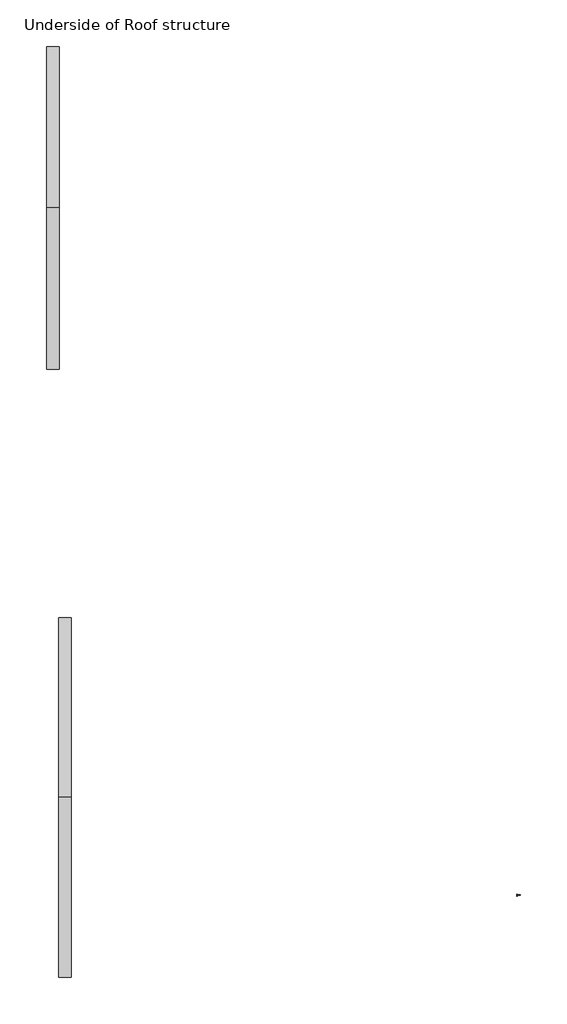
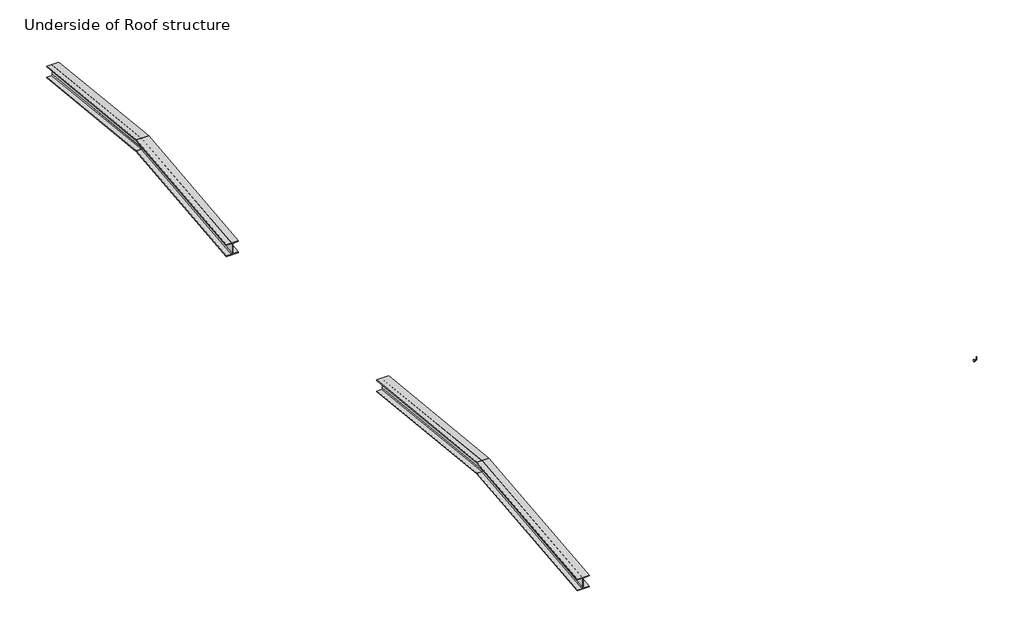
# One storey: 4 beams, 1 proxy.
"""IFC4 building model written with IfcOpenShell, lengths in millimetres."""

import ifcopenshell
import ifcopenshell.guid

model = None  # the IFC model being written
_history = None  # IfcOwnerHistory: only IFC2X3 demands one
_inside = {}  # id of a spatial element -> (the spatial element, [elements in it])
_under = {}  # id of a project, library or spatial element -> (it, [spatial elements below it])
_declared = {}  # id of a project -> (the project, [libraries it declares])
_typed = {}  # id of a type object -> (the type object, [elements of that type])
_made_of = {}  # id of a material, layer set ... -> (it, [elements and type objects made of it])


def new_model(schema):
    """Start an empty IFC model of exactly this schema.

    Asked for "IFC4X3", IfcOpenShell would pick the latest addendum, in which some entities
    have other attributes; the version numbers below select the first issue.
    IFC2X3 requires an IfcOwnerHistory on every rooted entity: one is made here for all.
    """
    global model, _history
    if schema == "IFC4X3":
        model = ifcopenshell.file(schema_version=(4, 3, 0, 0))
    else:
        model = ifcopenshell.file(schema=schema)
    _inside.clear()
    _under.clear()
    _declared.clear()
    _typed.clear()
    _made_of.clear()
    _history = None
    if model.schema == "IFC2X3":
        org = make("IfcOrganization", Name="unknown")
        user = make(
            "IfcPersonAndOrganization",
            ThePerson=make("IfcPerson", FamilyName="unknown"),
            TheOrganization=org,
        )
        app = make(
            "IfcApplication",
            ApplicationDeveloper=org,
            Version="unknown",
            ApplicationFullName="unknown",
            ApplicationIdentifier="unknown",
        )
        _history = make(
            "IfcOwnerHistory",
            OwningUser=user,
            OwningApplication=app,
            ChangeAction="ADDED",
            CreationDate=0,
        )
    return model


def make(cls, **values):
    """One entity of the class cls with the attributes given. An attribute that is None is left unset."""
    return model.create_entity(
        cls, **{name: value for name, value in values.items() if value is not None}
    )


def rooted(cls, **values):
    """An entity with a GlobalId (a new one), such as an element, a storey or a relation."""
    return make(cls, GlobalId=ifcopenshell.guid.new(), OwnerHistory=_history, **values)


def si_unit(unit_type, name, prefix=None):
    """IfcSIUnit, for example si_unit("LENGTHUNIT", "METRE", prefix="MILLI")."""
    return make("IfcSIUnit", UnitType=unit_type, Prefix=prefix, Name=name)


def assignment(units):
    """IfcUnitAssignment: the units of a project."""
    return None if units is None else make("IfcUnitAssignment", Units=units)


def point(xyz):
    """IfcCartesianPoint."""
    return None if xyz is None else make("IfcCartesianPoint", Coordinates=xyz)


def direction(xyz):
    """IfcDirection."""
    return None if xyz is None else make("IfcDirection", DirectionRatios=xyz)


def frame(location, z_axis=None, x_axis=None):
    """IfcAxis2Placement3D, a coordinate frame: its origin and axes. An axis left out is left unset."""
    return make(
        "IfcAxis2Placement3D",
        Location=point(location),
        Axis=direction(z_axis),
        RefDirection=direction(x_axis),
    )


def frame_2d(location, x_axis=None):
    """IfcAxis2Placement2D, a coordinate frame in the plane: its origin and x axis."""
    return make(
        "IfcAxis2Placement2D", Location=point(location), RefDirection=direction(x_axis)
    )


def origin():
    """The frame at (0, 0, 0) with its axes left unset."""
    return frame((0.0, 0.0, 0.0))


def origin_with_axes():
    """The frame at (0, 0, 0) with the z axis (0, 0, 1) and the x axis (1, 0, 0) written out."""
    return frame((0.0, 0.0, 0.0), z_axis=(0.0, 0.0, 1.0), x_axis=(1.0, 0.0, 0.0))


def place(relative_to, where):
    """IfcLocalPlacement: puts the frame where relative to a parent placement (None: the world)."""
    return make(
        "IfcLocalPlacement", PlacementRelTo=relative_to, RelativePlacement=where
    )


def context(
    kind, dimensions, precision=None, world=None, true_north=None, identifier=None
):
    """IfcGeometricRepresentationContext, for example the 3D "Model" context."""
    return make(
        "IfcGeometricRepresentationContext",
        ContextIdentifier=identifier,
        ContextType=kind,
        CoordinateSpaceDimension=dimensions,
        Precision=precision,
        WorldCoordinateSystem=world,
        TrueNorth=true_north,
    )


def project(units=None, contexts=None):
    """IfcProject with its units and contexts."""
    return rooted(
        "IfcProject",
        Name="project",
        RepresentationContexts=contexts,
        UnitsInContext=assignment(units),
    )


def spatial(cls, under=None, at=None, **own):
    """A site, building, storey or space (cls), placed at a placement, below another one or the project."""
    s = rooted(cls, ObjectPlacement=at, **own)
    if under is not None:
        _under.setdefault(under.id(), (under, []))[1].append(s)
    return s


def polyline(points):
    """IfcPolyline through the points."""
    return make("IfcPolyline", Points=[point(p) for p in points])


def circle_curve(where, radius):
    """IfcCircle in the frame where."""
    return make("IfcCircle", Position=where, Radius=radius)


def ellipse_curve(where, semi_axis1, semi_axis2):
    """IfcEllipse in the frame where."""
    return make(
        "IfcEllipse", Position=where, SemiAxis1=semi_axis1, SemiAxis2=semi_axis2
    )


def trimmed(basis, trim1, trim2, sense, master):
    """IfcTrimmedCurve: the piece of a basis curve between two trims."""
    return make(
        "IfcTrimmedCurve",
        BasisCurve=basis,
        Trim1=trim1,
        Trim2=trim2,
        SenseAgreement=sense,
        MasterRepresentation=master,
    )


def segment(curve, same_sense, transition):
    """IfcCompositeCurveSegment."""
    return make(
        "IfcCompositeCurveSegment",
        Transition=transition,
        SameSense=same_sense,
        ParentCurve=curve,
    )


def composite_curve(segments, self_intersect=None):
    """IfcCompositeCurve: segments joined end to end."""
    return make("IfcCompositeCurve", Segments=segments, SelfIntersect=self_intersect)


def outline(outer, holes=None, kind="AREA"):
    """IfcArbitraryClosedProfileDef: a profile drawn as a closed curve; with holes, ...WithVoids."""
    if holes is None:
        return make("IfcArbitraryClosedProfileDef", ProfileType=kind, OuterCurve=outer)
    return make(
        "IfcArbitraryProfileDefWithVoids",
        ProfileType=kind,
        OuterCurve=outer,
        InnerCurves=holes,
    )


def extrude(swept, where, along, depth):
    """IfcExtrudedAreaSolid: the profile swept, set in the frame where, extruded along a direction by depth."""
    return make(
        "IfcExtrudedAreaSolid",
        SweptArea=swept,
        Position=where,
        ExtrudedDirection=direction(along),
        Depth=depth,
    )


def shape(context_of_items, identifier, shape_type, items):
    """IfcShapeRepresentation: the items that make up one representation, for example the "Body"."""
    return make(
        "IfcShapeRepresentation",
        ContextOfItems=context_of_items,
        RepresentationIdentifier=identifier,
        RepresentationType=shape_type,
        Items=items,
    )


def source(mapping_origin, context_of_items, identifier, shape_type, items):
    """IfcRepresentationMap: a shape defined once, which mapped items show again and again."""
    return make(
        "IfcRepresentationMap",
        MappingOrigin=mapping_origin,
        MappedRepresentation=shape(context_of_items, identifier, shape_type, items),
    )


def transform(
    local_origin,
    x_axis=None,
    y_axis=None,
    z_axis=None,
    scale=None,
    scale2=None,
    scale3=None,
    uniform=True,
):
    """IfcCartesianTransformationOperator3D, or its non-uniform kind. x_axis, y_axis, z_axis: its Axis1, 2, 3."""
    if uniform:
        return make(
            "IfcCartesianTransformationOperator3D",
            Axis1=direction(x_axis),
            Axis2=direction(y_axis),
            LocalOrigin=point(local_origin),
            Scale=scale,
            Axis3=direction(z_axis),
        )
    return make(
        "IfcCartesianTransformationOperator3DnonUniform",
        Axis1=direction(x_axis),
        Axis2=direction(y_axis),
        LocalOrigin=point(local_origin),
        Scale=scale,
        Axis3=direction(z_axis),
        Scale2=scale2,
        Scale3=scale3,
    )


def mapped(mapping_source, mapping_target):
    """IfcMappedItem: shows the shape of a source again, moved by a transform."""
    return make(
        "IfcMappedItem", MappingSource=mapping_source, MappingTarget=mapping_target
    )


def made_of(thing, what):
    """Note that an element or type object is made of a material, layer set ...; save() writes the relation."""
    if what is not None:
        _made_of.setdefault(what.id(), (what, []))[1].append(thing)
    return thing


def element(
    cls,
    number,
    at=None,
    inside=None,
    cuts=None,
    type_object=None,
    material=None,
    context=None,
    identifier="Body",
    shape_type=None,
    held_by="IfcProductDefinitionShape",
    body=None,
    shapes=None,
    **own,
):
    """One element of the class cls, such as IfcWall. Its Tag is "e" and its number.

    at: its placement. inside: the storey or other place that contains it. cuts: it is an
    opening in that element (IfcRelVoidsElement). A single representation is given by context,
    identifier, shape_type and body (its items); several are given by shapes. held_by: the class
    of the entity that holds the representations. save() writes the other relations.
    """
    e = rooted(cls, Tag="e%d" % number, ObjectPlacement=at, **own)
    if body is not None:
        shapes = [shape(context, identifier, shape_type, body)]
    if shapes is not None:
        e.Representation = make(held_by, Representations=shapes)
    if inside is not None:
        _inside.setdefault(inside.id(), (inside, []))[1].append(e)
    if cuts is not None:
        rooted(
            "IfcRelVoidsElement", RelatingBuildingElement=cuts, RelatedOpeningElement=e
        )
    if type_object is not None:
        _typed.setdefault(type_object.id(), (type_object, []))[1].append(e)
    return made_of(e, material)


def aggregate(whole, parts):
    """IfcRelAggregates: a whole, such as a stair, and the parts it consists of."""
    return rooted("IfcRelAggregates", RelatingObject=whole, RelatedObjects=parts)


def save(model, path):
    """Write the relations noted so far, then the file.

    IfcRelAggregates (storeys below a building ...), IfcRelContainedInSpatialStructure (elements
    in a storey), IfcRelDefinesByType, IfcRelAssociatesMaterial and IfcRelDeclares: one each for
    every whole, place, type object, material and project.
    """
    for whole, parts in _under.values():
        aggregate(whole, parts)
    for where, things in _inside.values():
        rooted(
            "IfcRelContainedInSpatialStructure",
            RelatedElements=things,
            RelatingStructure=where,
        )
    for kind, things in _typed.values():
        rooted("IfcRelDefinesByType", RelatedObjects=things, RelatingType=kind)
    for what, things in _made_of.values():
        rooted("IfcRelAssociatesMaterial", RelatedObjects=things, RelatingMaterial=what)
    for by, libraries in _declared.values():
        rooted("IfcRelDeclares", RelatingContext=by, RelatedDefinitions=libraries)
    model.write(path)


def plane_surface(at):
    """IfcPlane: the flat surface through the origin of the frame at, square to its z axis."""
    return make("IfcPlane", Position=at)


def cylinder_surface(at, radius):
    """IfcCylindricalSurface: all points at the distance radius from the z axis of the frame at."""
    return make("IfcCylindricalSurface", Position=at, Radius=radius)


def revolved_surface(curve, axis_point, axis_direction):
    """IfcSurfaceOfRevolution: the curve turned about the line through axis_point along axis_direction."""
    return make(
        "IfcSurfaceOfRevolution",
        SweptCurve=make("IfcArbitraryOpenProfileDef", ProfileType="CURVE", Curve=curve),
        AxisPosition=make("IfcAxis1Placement", Location=point(axis_point), Axis=direction(axis_direction)),
    )


def advanced_brep(points, edges, surfaces, faces):
    """IfcAdvancedBrep: a solid bounded by faces that lie on surfaces and meet in shared edges.

    An edge is (start, end): straight between two places in points (the first is 0);
    or (start, end, curve); or (start, end, curve, False) where it runs against its curve.
    A face is (place in surfaces, loops), or (place, loops, False) where it looks against
    its surface's normal. A loop lists edges by number (the first is 1), with a minus sign
    where the edge is run from its end to its start. The first loop is the outer one.
    """
    corners = [point(p) for p in points]
    vertices = [make("IfcVertexPoint", VertexGeometry=c) for c in corners]
    made = []
    for start, end, *more in edges:
        made.append(
            make(
                "IfcEdgeCurve",
                EdgeStart=vertices[start],
                EdgeEnd=vertices[end],
                EdgeGeometry=more[0] if more else make("IfcPolyline", Points=[corners[start], corners[end]]),
                SameSense=more[1] if len(more) > 1 else True,
            )
        )
    hull = []
    for where, loops, *sense in faces:
        bounds = []
        for j, loop in enumerate(loops):
            ring = [make("IfcOrientedEdge", EdgeElement=made[abs(k) - 1], Orientation=k > 0) for k in loop]
            bounds.append(
                make(
                    "IfcFaceOuterBound" if j == 0 else "IfcFaceBound",
                    Bound=make("IfcEdgeLoop", EdgeList=ring),
                    Orientation=True,
                )
            )
        hull.append(make("IfcAdvancedFace", Bounds=bounds, FaceSurface=surfaces[where], SameSense=sense[0] if sense else True))
    return make("IfcAdvancedBrep", Outer=make("IfcClosedShell", CfsFaces=hull))


def support_metal_circular1_support_metal_circular_6fb01533(model_context):
    return source(origin(), model_context, "Body", "SolidModel", [
        advanced_brep(
        [(0.0, 63.5, -69.85), (0.0, 63.5, -82.55), (0.0, 12.7, -69.85), (0.0, 12.7, -82.55), (0.0, -6.35, -63.5), (0.0, 6.35, -63.5), (0.0, 6.35, 0.0), (0.0, -6.35, 0.0)],
        [
            (0, 1, circle_curve(frame((0.0, 63.5, -76.2), z_axis=(0.0, 1.0, 0.0), x_axis=(0.0, 0.0, -1.0)), 6.35)),
            (1, 0, circle_curve(frame((0.0, 63.5, -76.2), z_axis=(0.0, 1.0, 0.0), x_axis=(0.0, 0.0, -1.0)), 6.35)),
            (0, 2),
            (2, 3, circle_curve(frame((0.0, 12.7, -76.2), z_axis=(0.0, 1.0, 0.0), x_axis=(0.0, 0.0, -1.0)), 6.35)),
            (3, 1),
            (3, 2, circle_curve(frame((0.0, 12.7, -76.2), z_axis=(0.0, 1.0, 0.0), x_axis=(0.0, 0.0, -1.0)), 6.35)),
            (4, 3, circle_curve(frame((0.0, 12.7, -63.5), z_axis=(1.0, 0.0, 0.0), x_axis=(0.0, 0.0, -1.0)), 19.05)),
            (2, 5, circle_curve(frame((0.0, 12.7, -63.5), z_axis=(-1.0, 0.0, 0.0), x_axis=(0.0, 0.0, -1.0)), 6.35)),
            (5, 4, circle_curve(frame((0.0, 0.0, -63.5), z_axis=(0.0, 0.0, -1.0), x_axis=(0.0, -1.0, 0.0)), 6.35)),
            (4, 5, circle_curve(frame((0.0, 0.0, -63.5), z_axis=(0.0, 0.0, -1.0), x_axis=(0.0, -1.0, 0.0)), 6.35)),
            (6, 7, circle_curve(frame((0.0, 0.0, 0.0), z_axis=(0.0, 0.0, 1.0), x_axis=(0.0, -1.0, 0.0)), 6.35)),
            (7, 6, circle_curve(frame((0.0, 0.0, 0.0), z_axis=(0.0, 0.0, 1.0), x_axis=(0.0, -1.0, 0.0)), 6.35)),
            (5, 6),
            (7, 4),
        ],
        [
            plane_surface(frame((0.0, 63.5, -76.2), z_axis=(0.0, 1.0, 0.0), x_axis=(1.0, 0.0, 0.0))),
            cylinder_surface(frame((0.0, 63.5, -76.2), z_axis=(0.0, 1.0, 0.0), x_axis=(0.0, 0.0, -1.0)), 6.35),
            revolved_surface(trimmed(ellipse_curve(frame((0.0, 12.7, -76.2), z_axis=(0.0, 1.0, 0.0), x_axis=(0.0, 0.0, -1.0)), 6.35, 6.35), [point((0.0, 12.7, -69.85))], [point((0.0, 12.7, -82.55))], True, "CARTESIAN"), (0.0, 12.7, -63.5), (-1.0, 0.0, 0.0)),
            revolved_surface(trimmed(ellipse_curve(frame((0.0, 12.7, -76.2), z_axis=(0.0, 1.0, 0.0), x_axis=(0.0, 0.0, -1.0)), 6.35, 6.35), [point((0.0, 12.7, -82.55))], [point((0.0, 12.7, -69.85))], True, "CARTESIAN"), (0.0, 12.7, -63.5), (-1.0, 0.0, 0.0)),
            plane_surface(origin_with_axes()),
            cylinder_surface(frame((0.0, 0.0, -63.5), z_axis=(0.0, 0.0, -1.0), x_axis=(0.0, -1.0, 0.0)), 6.35),
        ],
        [
            (0, [[1, 2]]),
            (1, [[-1, 3, 4, 5]]),
            (1, [[-2, -5, 6, -3]]),
            (2, [[7, -4, 8, 9]]),
            (3, [[-8, -6, -7, 10]]),
            (4, [[11, 12]]),
            (5, [[-9, 13, -12, 14]]),
            (5, [[-10, -14, -11, -13]]),
        ],
    ),
        extrude(outline(composite_curve([segment(trimmed(circle_curve(frame_2d((-76.2, 0.0)), 25.4), [point((-76.2, -25.4))], [point((-76.2, 25.4))], False, "CARTESIAN"), True, "CONTINUOUS"), segment(trimmed(circle_curve(frame_2d((-76.2, 0.0)), 25.4), [point((-76.2, 25.4))], [point((-76.2, -25.4))], False, "CARTESIAN"), True, "CONTINUOUS")], self_intersect=False)), frame((0.0, 63.5, 0.0), z_axis=(0.0, 1.0, 0.0), x_axis=(0.0, 0.0, 1.0)), (0.0, 0.0, 1.0), 12.7),
    ])


model = new_model("IFC4")

# Units and contexts
model_context = context("Model", 3, world=origin())
ifc_project = project(units=[si_unit("LENGTHUNIT", "METRE", prefix="MILLI")], contexts=[model_context])

# Site, building, storey
site = spatial("IfcSite", under=ifc_project)
building = spatial("IfcBuilding", under=site)
storey = spatial("IfcBuildingStorey", under=building, Name="Underside of Roof structure", Elevation=34036.0)

# Beams
placement = place(None, origin())
element("IfcBeam", 1, ObjectType="W-Wide Flange : W12X79", at=placement, inside=storey, context=model_context, shape_type="AdvancedBrep", body=[
    advanced_brep(
    [(-21755.4154607, 20844.8695005, 33191.9562864), (-21630.3204607, 20844.8695005, 33191.9562864), (-21607.7144607, 20844.8695005, 33214.6883829), (-21607.7144607, 20844.8695005, 33448.3947677), (-21630.3204607, 20844.8695005, 33471.1268642), (-21755.4154607, 20844.8695005, 33471.1268642), (-21755.4154607, 20844.8695005, 33489.9), (-21448.0754607, 20844.8695005, 33489.9), (-21448.0754607, 20844.8695005, 33471.1268642), (-21573.1704607, 20844.8695005, 33471.1268642), (-21595.7764607, 20844.8695005, 33448.3947677), (-21595.7764607, 20844.8695005, 33214.6883829), (-21573.1704607, 20844.8695005, 33191.9562864), (-21448.0754607, 20844.8695005, 33191.9562864), (-21448.0754607, 20844.8695005, 33173.1831506), (-21755.4154607, 20844.8695005, 33173.1831506), (-21755.4154607, 16882.4695005, 33611.0562864), (-21630.3204607, 16882.4695005, 33611.0562864), (-21755.4154607, 16882.4695005, 33592.2831506), (-21448.0754607, 16882.4695005, 33592.2831506), (-21448.0754607, 16882.4695005, 33611.0562864), (-21573.1704607, 16882.4695005, 33611.0562864), (-21595.7764607, 16882.4695005, 33633.7883829), (-21595.7764607, 16882.4695005, 33867.4947677), (-21573.1704607, 16882.4695005, 33890.2268642), (-21448.0754607, 16882.4695005, 33890.2268642), (-21448.0754607, 16882.4695005, 33909.0), (-21755.4154607, 16882.4695005, 33909.0), (-21755.4154607, 16882.4695005, 33890.2268642), (-21630.3204607, 16882.4695005, 33890.2268642), (-21607.7144607, 16882.4695005, 33867.4947677), (-21607.7144607, 16882.4695005, 33633.7883829)],
    [
        (0, 1),
        (1, 2, ellipse_curve(frame((-21630.3204607, 20844.8695005, 33214.6883829), z_axis=(0.0, -1.0, 0.0), x_axis=(0.0, 0.0, 0.9999999999999999)), 22.7320964, 22.606)),
        (2, 3),
        (3, 4, ellipse_curve(frame((-21630.3204607, 20844.8695005, 33448.3947677), z_axis=(0.0, -1.0, 0.0), x_axis=(0.0, 0.0, 0.9999999999999999)), 22.7320964, 22.606)),
        (4, 5),
        (5, 6),
        (6, 7),
        (7, 8),
        (8, 9),
        (9, 10, ellipse_curve(frame((-21573.1704607, 20844.8695005, 33448.3947677), z_axis=(0.0, -1.0, 0.0), x_axis=(0.0, 0.0, 0.9999999999999999)), 22.7320964, 22.606)),
        (10, 11),
        (11, 12, ellipse_curve(frame((-21573.1704607, 20844.8695005, 33214.6883829), z_axis=(0.0, -1.0, 0.0), x_axis=(0.0, 0.0, 0.9999999999999999)), 22.7320964, 22.606)),
        (12, 13),
        (13, 14),
        (14, 15),
        (15, 0),
        (0, 16),
        (16, 17),
        (17, 1),
        (15, 18),
        (18, 16),
        (18, 19),
        (19, 20),
        (20, 21),
        (21, 22, ellipse_curve(frame((-21573.1704607, 16882.4695005, 33633.7883829), z_axis=(0.0, 1.0, 0.0), x_axis=(0.0, 0.0, 0.9999999999999999)), 22.7320964, 22.606)),
        (22, 23),
        (23, 24, ellipse_curve(frame((-21573.1704607, 16882.4695005, 33867.4947677), z_axis=(0.0, 1.0, 0.0), x_axis=(0.0, 0.0, 0.9999999999999999)), 22.7320964, 22.606)),
        (24, 25),
        (25, 26),
        (26, 27),
        (27, 28),
        (28, 29),
        (29, 30, ellipse_curve(frame((-21630.3204607, 16882.4695005, 33867.4947677), z_axis=(0.0, 1.0, 0.0), x_axis=(0.0, 0.0, 0.9999999999999999)), 22.7320964, 22.606)),
        (30, 31),
        (31, 17, ellipse_curve(frame((-21630.3204607, 16882.4695005, 33633.7883829), z_axis=(0.0, 1.0, 0.0), x_axis=(0.0, 0.0, 0.9999999999999999)), 22.7320964, 22.606)),
        (31, 2),
        (30, 3),
        (29, 4),
        (28, 5),
        (27, 6),
        (26, 7),
        (25, 8),
        (24, 9),
        (23, 10),
        (22, 11),
        (21, 12),
        (20, 13),
        (19, 14),
    ],
    [
        plane_surface(frame((-23272.9998994, 20844.8695005, 33801.3683204), z_axis=(0.0, 1.0, 0.0), x_axis=(0.0, 0.0, 1.0))),
        plane_surface(frame((-21692.8679607, 20969.2190095, 33178.8039345), z_axis=(0.0, 0.10518252182083103, 0.9944529335787644), x_axis=(1.0, 0.0, 0.0))),
        plane_surface(frame((-21755.4154607, 20968.2371832, 33169.5212136), z_axis=(-1.0, 0.0, 0.0), x_axis=(0.0, 0.10518252182083183, 0.9944529335787644))),
        plane_surface(frame((-21601.7454607, 16882.4695005, 33592.2831506), z_axis=(0.0, -1.0, 0.0), x_axis=(0.0, 0.0, 1.0))),
        revolved_surface(polyline([(-21607.7144607, 16880.091744411304, 33634.03987627958), (-21607.7144607, 20847.247256588096, 33214.43688941473)]), (-21630.3204607, 20971.5967656, 33201.2845375), (0.0, -0.9944529335787643, 0.10518252182083102)),
        plane_surface(frame((-21607.7144607, 20983.8195005, 33316.8449407), z_axis=(-1.0, 0.0, 0.0), x_axis=(0.0, 0.10518252182083183, 0.9944529335787644))),
        revolved_surface(polyline([(-21630.3204607, 16882.46950049405, 33890.226864143755), (-21630.3204607, 20849.625012670844, 33470.6238772789)]), (-21630.3204607, 20996.0422355, 33432.4053438), (0.0, -0.9944529335787643, 0.10518252182083102)),
        plane_surface(frame((-21692.8679607, 20998.4199915, 33454.8859468), z_axis=(0.0, -0.10518252182083103, -0.9944529335787644), x_axis=(-1.0, 0.0, 0.0))),
        plane_surface(frame((-21755.4154607, 20999.4018178, 33464.1686678), z_axis=(-1.0, 0.0, 0.0), x_axis=(0.0, 0.10518252182083183, 0.9944529335787644))),
        plane_surface(frame((-21601.7454607, 21000.383644, 33473.4513887), z_axis=(0.0, 0.10518252182083103, 0.9944529335787644), x_axis=(1.0, 0.0, 0.0))),
        plane_surface(frame((-21448.0754607, 20999.4018178, 33464.1686678), z_axis=(1.0, 0.0, 0.0), x_axis=(0.0, -0.10518252182083183, -0.9944529335787644))),
        plane_surface(frame((-21510.6229607, 20998.4199915, 33454.8859468), z_axis=(0.0, -0.10518252182083103, -0.9944529335787644), x_axis=(-1.0, 0.0, 0.0))),
        revolved_surface(polyline([(-21595.7764607, 16880.09174440577, 33867.74626112727), (-21595.7764607, 20847.247256582563, 33448.14327426242)]), (-21573.1704607, 20996.0422355, 33432.4053438), (0.0, -0.9944529335787643, 0.10518252182083102)),
        plane_surface(frame((-21595.7764607, 20983.8195005, 33316.8449407), z_axis=(1.0, 0.0, 0.0), x_axis=(0.0, -0.10518252182083183, -0.9944529335787644))),
        revolved_surface(polyline([(-21573.1704607, 16877.713988323023, 33611.5592732631), (-21573.1704607, 20844.869500499815, 33191.95628639824)]), (-21573.1704607, 20971.5967656, 33201.2845375), (0.0, -0.9944529335787643, 0.10518252182083102)),
        plane_surface(frame((-21510.6229607, 20969.2190095, 33178.8039345), z_axis=(0.0, 0.10518252182083103, 0.9944529335787644), x_axis=(1.0, 0.0, 0.0))),
        plane_surface(frame((-21448.0754607, 20968.2371832, 33169.5212136), z_axis=(1.0, 0.0, 0.0), x_axis=(0.0, -0.10518252182083183, -0.9944529335787644))),
        plane_surface(frame((-21601.7454607, 20967.255357, 33160.2384927), z_axis=(0.0, -0.10518252182083103, -0.9944529335787644), x_axis=(-1.0, 0.0, 0.0))),
    ],
    [
        (0, [[1, 2, 3, 4, 5, 6, 7, 8, 9, 10, 11, 12, 13, 14, 15, 16]]),
        (1, [[17, 18, 19, -1]]),
        (2, [[20, 21, -17, -16]]),
        (3, [[-21, 22, 23, 24, 25, 26, 27, 28, 29, 30, 31, 32, 33, 34, 35, -18]]),
        (4, [[-19, -35, 36, -2]]),
        (5, [[-36, -34, 37, -3]]),
        (6, [[-37, -33, 38, -4]]),
        (7, [[-38, -32, 39, -5]]),
        (8, [[-39, -31, 40, -6]]),
        (9, [[-40, -30, 41, -7]]),
        (10, [[-41, -29, 42, -8]]),
        (11, [[-42, -28, 43, -9]]),
        (12, [[-43, -27, 44, -10]]),
        (13, [[-44, -26, 45, -11]]),
        (14, [[-45, -25, 46, -12]]),
        (15, [[-46, -24, 47, -13]]),
        (16, [[-47, -23, 48, -14]]),
        (17, [[-48, -22, -20, -15]]),
    ],
),
])
element("IfcBeam", 2, ObjectType="W-Wide Flange : W12X79", at=placement, inside=storey, context=model_context, shape_type="AdvancedBrep", body=[
    advanced_brep(
    [(-21630.3204607, 12920.0695005, 33191.9562864), (-21755.4154607, 12920.0695005, 33191.9562864), (-21755.4154607, 12920.0695005, 33173.1831506), (-21448.0754607, 12920.0695005, 33173.1831506), (-21448.0754607, 12920.0695005, 33191.9562864), (-21573.1704607, 12920.0695005, 33191.9562864), (-21595.7764607, 12920.0695005, 33214.6883829), (-21595.7764607, 12920.0695005, 33448.3947677), (-21573.1704607, 12920.0695005, 33471.1268642), (-21448.0754607, 12920.0695005, 33471.1268642), (-21448.0754607, 12920.0695005, 33489.9), (-21755.4154607, 12920.0695005, 33489.9), (-21755.4154607, 12920.0695005, 33471.1268642), (-21630.3204607, 12920.0695005, 33471.1268642), (-21607.7144607, 12920.0695005, 33448.3947677), (-21607.7144607, 12920.0695005, 33214.6883829), (-21607.7144607, 16882.4695005, 33633.7883829), (-21630.3204607, 16882.4695005, 33611.0562864), (-21755.4154607, 16882.4695005, 33611.0562864), (-21607.7144607, 16882.4695005, 33867.4947677), (-21630.3204607, 16882.4695005, 33890.2268642), (-21755.4154607, 16882.4695005, 33890.2268642), (-21755.4154607, 16882.4695005, 33909.0), (-21448.0754607, 16882.4695005, 33909.0), (-21448.0754607, 16882.4695005, 33890.2268642), (-21573.1704607, 16882.4695005, 33890.2268642), (-21595.7764607, 16882.4695005, 33867.4947677), (-21595.7764607, 16882.4695005, 33633.7883829), (-21573.1704607, 16882.4695005, 33611.0562864), (-21448.0754607, 16882.4695005, 33611.0562864), (-21448.0754607, 16882.4695005, 33592.2831506), (-21755.4154607, 16882.4695005, 33592.2831506)],
    [
        (0, 1),
        (1, 2),
        (2, 3),
        (3, 4),
        (4, 5),
        (5, 6, ellipse_curve(frame((-21573.1704607, 12920.0695005, 33214.6883829), z_axis=(0.0, 1.0, 0.0), x_axis=(0.0, 0.0, 1.0)), 22.7320964, 22.606)),
        (6, 7),
        (7, 8, ellipse_curve(frame((-21573.1704607, 12920.0695005, 33448.3947677), z_axis=(0.0, 1.0, 0.0), x_axis=(0.0, 0.0, 1.0)), 22.7320964, 22.606)),
        (8, 9),
        (9, 10),
        (10, 11),
        (11, 12),
        (12, 13),
        (13, 14, ellipse_curve(frame((-21630.3204607, 12920.0695005, 33448.3947677), z_axis=(0.0, 1.0, 0.0), x_axis=(0.0, 0.0, 1.0)), 22.7320964, 22.606)),
        (14, 15),
        (15, 0, ellipse_curve(frame((-21630.3204607, 12920.0695005, 33214.6883829), z_axis=(0.0, 1.0, 0.0), x_axis=(0.0, 0.0, 1.0)), 22.7320964, 22.606)),
        (15, 16),
        (16, 17, ellipse_curve(frame((-21630.3204607, 16882.4695005, 33633.7883829), z_axis=(0.0, 1.0, 0.0), x_axis=(0.0, 0.0, 1.0)), 22.7320964, 22.606)),
        (17, 0),
        (17, 18),
        (18, 1),
        (16, 19),
        (19, 20, ellipse_curve(frame((-21630.3204607, 16882.4695005, 33867.4947677), z_axis=(0.0, -1.0, 0.0), x_axis=(0.0, 0.0, 1.0)), 22.7320964, 22.606)),
        (20, 21),
        (21, 22),
        (22, 23),
        (23, 24),
        (24, 25),
        (25, 26, ellipse_curve(frame((-21573.1704607, 16882.4695005, 33867.4947677), z_axis=(0.0, -1.0, 0.0), x_axis=(0.0, 0.0, 1.0)), 22.7320964, 22.606)),
        (26, 27),
        (27, 28, ellipse_curve(frame((-21573.1704607, 16882.4695005, 33633.7883829), z_axis=(0.0, -1.0, 0.0), x_axis=(0.0, 0.0, 1.0)), 22.7320964, 22.606)),
        (28, 29),
        (29, 30),
        (30, 31),
        (31, 18),
        (31, 2),
        (14, 19),
        (13, 20),
        (12, 21),
        (11, 22),
        (10, 23),
        (9, 24),
        (8, 25),
        (7, 26),
        (6, 27),
        (5, 28),
        (4, 29),
        (3, 30),
    ],
    [
        plane_surface(frame((-23272.9998994, 12920.0695005, 33801.3683204), z_axis=(0.0, -1.0, 0.0), x_axis=(0.0, 0.0, 1.0))),
        revolved_surface(polyline([(-21607.7144607, 16884.847256589805, 33634.03987626912), (-21607.7144607, 12917.69174441301, 33214.436889404264)]), (-21630.3204607, 12793.3422355, 33201.2845375), (0.0, 0.9944529335787644, 0.10518252182083103)),
        plane_surface(frame((-21692.8679607, 12795.7199915, 33178.8039345), z_axis=(0.0, -0.10518252182083103, 0.9944529335787644), x_axis=(1.0, 0.0, 0.0))),
        plane_surface(frame((-21601.7454607, 16882.4695005, 33592.2831506), z_axis=(0.0, 1.0, 0.0), x_axis=(0.0, 0.0, -1.0))),
        plane_surface(frame((-21755.4154607, 12796.7018178, 33169.5212136), z_axis=(-1.0, 0.0, 0.0), x_axis=(0.0, -0.10518252182083185, 0.9944529335787644))),
        plane_surface(frame((-21607.7144607, 12781.1195005, 33316.8449407), z_axis=(-1.0, 0.0, 0.0), x_axis=(0.0, -0.10518252182083185, 0.9944529335787644))),
        revolved_surface(polyline([(-21630.3204607, 16882.469500507057, 33890.2268641333), (-21630.3204607, 12915.313988330263, 33470.623877268445)]), (-21630.3204607, 12768.8967656, 33432.4053438), (0.0, 0.9944529335787644, 0.10518252182083103)),
        plane_surface(frame((-21692.8679607, 12766.5190095, 33454.8859468), z_axis=(0.0, 0.10518252182083103, -0.9944529335787644), x_axis=(-1.0, 0.0, 0.0))),
        plane_surface(frame((-21755.4154607, 12765.5371832, 33464.1686678), z_axis=(-1.0, 0.0, 0.0), x_axis=(0.0, -0.10518252182083185, 0.9944529335787644))),
        plane_surface(frame((-21601.7454607, 12764.555357, 33473.4513887), z_axis=(0.0, -0.10518252182083103, 0.9944529335787644), x_axis=(1.0, 0.0, 0.0))),
        plane_surface(frame((-21448.0754607, 12765.5371832, 33464.1686678), z_axis=(1.0, 0.0, 0.0), x_axis=(0.0, 0.10518252182083185, -0.9944529335787644))),
        plane_surface(frame((-21510.6229607, 12766.5190095, 33454.8859468), z_axis=(0.0, 0.10518252182083103, -0.9944529335787644), x_axis=(-1.0, 0.0, 0.0))),
        revolved_surface(polyline([(-21595.7764607, 16884.847256595338, 33867.746261116816), (-21595.7764607, 12917.691744418544, 33448.14327425196)]), (-21573.1704607, 12768.8967656, 33432.4053438), (0.0, 0.9944529335787644, 0.10518252182083103)),
        plane_surface(frame((-21595.7764607, 12781.1195005, 33316.8449407), z_axis=(1.0, 0.0, 0.0), x_axis=(0.0, 0.10518252182083185, -0.9944529335787644))),
        revolved_surface(polyline([(-21573.1704607, 16887.225012678085, 33611.559273252635), (-21573.1704607, 12920.069500501291, 33191.95628638778)]), (-21573.1704607, 12793.3422355, 33201.2845375), (0.0, 0.9944529335787644, 0.10518252182083103)),
        plane_surface(frame((-21510.6229607, 12795.7199915, 33178.8039345), z_axis=(0.0, -0.10518252182083103, 0.9944529335787644), x_axis=(1.0, 0.0, 0.0))),
        plane_surface(frame((-21448.0754607, 12796.7018178, 33169.5212136), z_axis=(1.0, 0.0, 0.0), x_axis=(0.0, 0.10518252182083185, -0.9944529335787644))),
        plane_surface(frame((-21601.7454607, 12797.683644, 33160.2384927), z_axis=(0.0, 0.10518252182083103, -0.9944529335787644), x_axis=(-1.0, 0.0, 0.0))),
    ],
    [
        (0, [[1, 2, 3, 4, 5, 6, 7, 8, 9, 10, 11, 12, 13, 14, 15, 16]]),
        (1, [[17, 18, 19, -16]]),
        (2, [[-19, 20, 21, -1]]),
        (3, [[-20, -18, 22, 23, 24, 25, 26, 27, 28, 29, 30, 31, 32, 33, 34, 35]]),
        (4, [[-21, -35, 36, -2]]),
        (5, [[37, -22, -17, -15]]),
        (6, [[38, -23, -37, -14]]),
        (7, [[39, -24, -38, -13]]),
        (8, [[40, -25, -39, -12]]),
        (9, [[41, -26, -40, -11]]),
        (10, [[42, -27, -41, -10]]),
        (11, [[43, -28, -42, -9]]),
        (12, [[44, -29, -43, -8]]),
        (13, [[45, -30, -44, -7]]),
        (14, [[46, -31, -45, -6]]),
        (15, [[47, -32, -46, -5]]),
        (16, [[48, -33, -47, -4]]),
        (17, [[-36, -34, -48, -3]]),
    ],
),
])
element("IfcBeam", 3, ObjectType="W-Wide Flange : W12X79", at=placement, inside=storey, context=model_context, shape_type="AdvancedBrep", body=[
    advanced_brep(
    [(-21450.6154607, 6824.0695005, 33143.5985941), (-21325.5204607, 6824.0695005, 33143.5985941), (-21302.9144607, 6824.0695005, 33166.3306906), (-21302.9144607, 6824.0695005, 33400.0370754), (-21325.5204607, 6824.0695005, 33422.7691719), (-21450.6154607, 6824.0695005, 33422.7691719), (-21450.6154607, 6824.0695005, 33441.5423077), (-21143.2754607, 6824.0695005, 33441.5423077), (-21143.2754607, 6824.0695005, 33422.7691719), (-21268.3704607, 6824.0695005, 33422.7691719), (-21290.9764607, 6824.0695005, 33400.0370754), (-21290.9764607, 6824.0695005, 33166.3306906), (-21268.3704607, 6824.0695005, 33143.5985941), (-21143.2754607, 6824.0695005, 33143.5985941), (-21143.2754607, 6824.0695005, 33124.8254583), (-21450.6154607, 6824.0695005, 33124.8254583), (-21450.6154607, 2404.4695005, 33611.0562864), (-21325.5204607, 2404.4695005, 33611.0562864), (-21450.6154607, 2404.4695005, 33592.2831506), (-21143.2754607, 2404.4695005, 33592.2831506), (-21143.2754607, 2404.4695005, 33611.0562864), (-21268.3704607, 2404.4695005, 33611.0562864), (-21290.9764607, 2404.4695005, 33633.7883829), (-21290.9764607, 2404.4695005, 33867.4947677), (-21268.3704607, 2404.4695005, 33890.2268642), (-21143.2754607, 2404.4695005, 33890.2268642), (-21143.2754607, 2404.4695005, 33909.0), (-21450.6154607, 2404.4695005, 33909.0), (-21450.6154607, 2404.4695005, 33890.2268642), (-21325.5204607, 2404.4695005, 33890.2268642), (-21302.9144607, 2404.4695005, 33867.4947677), (-21302.9144607, 2404.4695005, 33633.7883829)],
    [
        (0, 1),
        (1, 2, ellipse_curve(frame((-21325.5204607, 6824.0695005, 33166.3306906), z_axis=(0.0, -1.0, 0.0), x_axis=(0.0, 0.0, 0.9999999999999999)), 22.7320964, 22.606)),
        (2, 3),
        (3, 4, ellipse_curve(frame((-21325.5204607, 6824.0695005, 33400.0370754), z_axis=(0.0, -1.0, 0.0), x_axis=(0.0, 0.0, 0.9999999999999999)), 22.7320964, 22.606)),
        (4, 5),
        (5, 6),
        (6, 7),
        (7, 8),
        (8, 9),
        (9, 10, ellipse_curve(frame((-21268.3704607, 6824.0695005, 33400.0370754), z_axis=(0.0, -1.0, 0.0), x_axis=(0.0, 0.0, 0.9999999999999999)), 22.7320964, 22.606)),
        (10, 11),
        (11, 12, ellipse_curve(frame((-21268.3704607, 6824.0695005, 33166.3306906), z_axis=(0.0, -1.0, 0.0), x_axis=(0.0, 0.0, 0.9999999999999999)), 22.7320964, 22.606)),
        (12, 13),
        (13, 14),
        (14, 15),
        (15, 0),
        (0, 16),
        (16, 17),
        (17, 1),
        (15, 18),
        (18, 16),
        (18, 19),
        (19, 20),
        (20, 21),
        (21, 22, ellipse_curve(frame((-21268.3704607, 2404.4695005, 33633.7883829), z_axis=(0.0, 1.0, 0.0), x_axis=(0.0, 0.0, 0.9999999999999999)), 22.7320964, 22.606)),
        (22, 23),
        (23, 24, ellipse_curve(frame((-21268.3704607, 2404.4695005, 33867.4947677), z_axis=(0.0, 1.0, 0.0), x_axis=(0.0, 0.0, 0.9999999999999999)), 22.7320964, 22.606)),
        (24, 25),
        (25, 26),
        (26, 27),
        (27, 28),
        (28, 29),
        (29, 30, ellipse_curve(frame((-21325.5204607, 2404.4695005, 33867.4947677), z_axis=(0.0, 1.0, 0.0), x_axis=(0.0, 0.0, 0.9999999999999999)), 22.7320964, 22.606)),
        (30, 31),
        (31, 17, ellipse_curve(frame((-21325.5204607, 2404.4695005, 33633.7883829), z_axis=(0.0, 1.0, 0.0), x_axis=(0.0, 0.0, 0.9999999999999999)), 22.7320964, 22.606)),
        (31, 2),
        (30, 3),
        (29, 4),
        (28, 5),
        (27, 6),
        (26, 7),
        (25, 8),
        (24, 9),
        (23, 10),
        (22, 11),
        (21, 12),
        (20, 13),
        (19, 14),
    ],
    [
        plane_surface(frame((-23272.9998994, 6824.0695005, 33801.3683204), z_axis=(0.0, 1.0, 0.0), x_axis=(0.0, 0.0, 1.0))),
        plane_surface(frame((-21388.0679607, 6948.4190095, 33130.4462422), z_axis=(0.0, 0.10518252182083103, 0.9944529335787644), x_axis=(1.0, 0.0, 0.0))),
        plane_surface(frame((-21450.6154607, 6947.4371832, 33121.1635213), z_axis=(-1.0, 0.0, 0.0), x_axis=(0.0, 0.10518252182083125, 0.9944529335787644))),
        plane_surface(frame((-21296.9454607, 2404.4695005, 33592.2831506), z_axis=(0.0, -1.0, 0.0), x_axis=(0.0, 0.0, 1.0))),
        revolved_surface(polyline([(-21302.9144607, 2402.091744412107, 33634.039876287185), (-21302.9144607, 6826.447256588095, 33166.07919711473)]), (-21325.5204607, 6950.7967656, 33152.9268452), (0.0, -0.9944529335787643, 0.10518252182083102)),
        plane_surface(frame((-21302.9144607, 6963.0195005, 33268.4872484), z_axis=(-1.0, 0.0, 0.0), x_axis=(0.0, 0.10518252182083125, 0.9944529335787644))),
        revolved_surface(polyline([(-21325.5204607, 2404.4695004948553, 33890.226864151366), (-21325.5204607, 6828.825012670844, 33422.2661849789)]), (-21325.5204607, 6975.2422355, 33384.0476515), (0.0, -0.9944529335787643, 0.10518252182083102)),
        plane_surface(frame((-21388.0679607, 6977.6199915, 33406.5282545), z_axis=(0.0, -0.10518252182083103, -0.9944529335787644), x_axis=(-1.0, 0.0, 0.0))),
        plane_surface(frame((-21450.6154607, 6978.6018178, 33415.8109754), z_axis=(-1.0, 0.0, 0.0), x_axis=(0.0, 0.10518252182083125, 0.9944529335787644))),
        plane_surface(frame((-21296.9454607, 6979.583644, 33425.0936964), z_axis=(0.0, 0.10518252182083103, 0.9944529335787644), x_axis=(1.0, 0.0, 0.0))),
        plane_surface(frame((-21143.2754607, 6978.6018178, 33415.8109754), z_axis=(1.0, 0.0, 0.0), x_axis=(0.0, -0.10518252182083125, -0.9944529335787644))),
        plane_surface(frame((-21205.8229607, 6977.6199915, 33406.5282545), z_axis=(0.0, -0.10518252182083103, -0.9944529335787644), x_axis=(-1.0, 0.0, 0.0))),
        revolved_surface(polyline([(-21290.9764607, 2402.0917444065735, 33867.74626113488), (-21290.9764607, 6826.447256582563, 33399.78558196242)]), (-21268.3704607, 6975.2422355, 33384.0476515), (0.0, -0.9944529335787643, 0.10518252182083102)),
        plane_surface(frame((-21290.9764607, 6963.0195005, 33268.4872484), z_axis=(1.0, 0.0, 0.0), x_axis=(0.0, -0.10518252182083125, -0.9944529335787644))),
        revolved_surface(polyline([(-21268.3704607, 2399.713988323825, 33611.5592732707), (-21268.3704607, 6824.069500499813, 33143.59859409824)]), (-21268.3704607, 6950.7967656, 33152.9268452), (0.0, -0.9944529335787643, 0.10518252182083102)),
        plane_surface(frame((-21205.8229607, 6948.4190095, 33130.4462422), z_axis=(0.0, 0.10518252182083103, 0.9944529335787644), x_axis=(1.0, 0.0, 0.0))),
        plane_surface(frame((-21143.2754607, 6947.4371832, 33121.1635213), z_axis=(1.0, 0.0, 0.0), x_axis=(0.0, -0.10518252182083125, -0.9944529335787644))),
        plane_surface(frame((-21296.9454607, 6946.455357, 33111.8808004), z_axis=(0.0, -0.10518252182083103, -0.9944529335787644), x_axis=(-1.0, 0.0, 0.0))),
    ],
    [
        (0, [[1, 2, 3, 4, 5, 6, 7, 8, 9, 10, 11, 12, 13, 14, 15, 16]]),
        (1, [[17, 18, 19, -1]]),
        (2, [[20, 21, -17, -16]]),
        (3, [[-21, 22, 23, 24, 25, 26, 27, 28, 29, 30, 31, 32, 33, 34, 35, -18]]),
        (4, [[-19, -35, 36, -2]]),
        (5, [[-36, -34, 37, -3]]),
        (6, [[-37, -33, 38, -4]]),
        (7, [[-38, -32, 39, -5]]),
        (8, [[-39, -31, 40, -6]]),
        (9, [[-40, -30, 41, -7]]),
        (10, [[-41, -29, 42, -8]]),
        (11, [[-42, -28, 43, -9]]),
        (12, [[-43, -27, 44, -10]]),
        (13, [[-44, -26, 45, -11]]),
        (14, [[-45, -25, 46, -12]]),
        (15, [[-46, -24, 47, -13]]),
        (16, [[-47, -23, 48, -14]]),
        (17, [[-48, -22, -20, -15]]),
    ],
),
])
element("IfcBeam", 4, ObjectType="W-Wide Flange : W12X79", at=placement, inside=storey, context=model_context, shape_type="AdvancedBrep", body=[
    advanced_brep(
    [(-21325.5204607, -2015.1304995, 33143.5985941), (-21450.6154607, -2015.1304995, 33143.5985941), (-21450.6154607, -2015.1304995, 33124.8254583), (-21143.2754607, -2015.1304995, 33124.8254583), (-21143.2754607, -2015.1304995, 33143.5985941), (-21268.3704607, -2015.1304995, 33143.5985941), (-21290.9764607, -2015.1304995, 33166.3306906), (-21290.9764607, -2015.1304995, 33400.0370754), (-21268.3704607, -2015.1304995, 33422.7691719), (-21143.2754607, -2015.1304995, 33422.7691719), (-21143.2754607, -2015.1304995, 33441.5423077), (-21450.6154607, -2015.1304995, 33441.5423077), (-21450.6154607, -2015.1304995, 33422.7691719), (-21325.5204607, -2015.1304995, 33422.7691719), (-21302.9144607, -2015.1304995, 33400.0370754), (-21302.9144607, -2015.1304995, 33166.3306906), (-21302.9144607, 2404.4695005, 33633.7883829), (-21325.5204607, 2404.4695005, 33611.0562864), (-21450.6154607, 2404.4695005, 33611.0562864), (-21302.9144607, 2404.4695005, 33867.4947677), (-21325.5204607, 2404.4695005, 33890.2268642), (-21450.6154607, 2404.4695005, 33890.2268642), (-21450.6154607, 2404.4695005, 33909.0), (-21143.2754607, 2404.4695005, 33909.0), (-21143.2754607, 2404.4695005, 33890.2268642), (-21268.3704607, 2404.4695005, 33890.2268642), (-21290.9764607, 2404.4695005, 33867.4947677), (-21290.9764607, 2404.4695005, 33633.7883829), (-21268.3704607, 2404.4695005, 33611.0562864), (-21143.2754607, 2404.4695005, 33611.0562864), (-21143.2754607, 2404.4695005, 33592.2831506), (-21450.6154607, 2404.4695005, 33592.2831506)],
    [
        (0, 1),
        (1, 2),
        (2, 3),
        (3, 4),
        (4, 5),
        (5, 6, ellipse_curve(frame((-21268.3704607, -2015.1304995, 33166.3306906), z_axis=(0.0, 1.0, 0.0), x_axis=(0.0, 0.0, 1.0)), 22.7320964, 22.606)),
        (6, 7),
        (7, 8, ellipse_curve(frame((-21268.3704607, -2015.1304995, 33400.0370754), z_axis=(0.0, 1.0, 0.0), x_axis=(0.0, 0.0, 1.0)), 22.7320964, 22.606)),
        (8, 9),
        (9, 10),
        (10, 11),
        (11, 12),
        (12, 13),
        (13, 14, ellipse_curve(frame((-21325.5204607, -2015.1304995, 33400.0370754), z_axis=(0.0, 1.0, 0.0), x_axis=(0.0, 0.0, 1.0)), 22.7320964, 22.606)),
        (14, 15),
        (15, 0, ellipse_curve(frame((-21325.5204607, -2015.1304995, 33166.3306906), z_axis=(0.0, 1.0, 0.0), x_axis=(0.0, 0.0, 1.0)), 22.7320964, 22.606)),
        (15, 16),
        (16, 17, ellipse_curve(frame((-21325.5204607, 2404.4695005, 33633.7883829), z_axis=(0.0, 1.0, 0.0), x_axis=(0.0, 0.0, 1.0)), 22.7320964, 22.606)),
        (17, 0),
        (17, 18),
        (18, 1),
        (16, 19),
        (19, 20, ellipse_curve(frame((-21325.5204607, 2404.4695005, 33867.4947677), z_axis=(0.0, -1.0, 0.0), x_axis=(0.0, 0.0, 1.0)), 22.7320964, 22.606)),
        (20, 21),
        (21, 22),
        (22, 23),
        (23, 24),
        (24, 25),
        (25, 26, ellipse_curve(frame((-21268.3704607, 2404.4695005, 33867.4947677), z_axis=(0.0, -1.0, 0.0), x_axis=(0.0, 0.0, 1.0)), 22.7320964, 22.606)),
        (26, 27),
        (27, 28, ellipse_curve(frame((-21268.3704607, 2404.4695005, 33633.7883829), z_axis=(0.0, -1.0, 0.0), x_axis=(0.0, 0.0, 1.0)), 22.7320964, 22.606)),
        (28, 29),
        (29, 30),
        (30, 31),
        (31, 18),
        (31, 2),
        (14, 19),
        (13, 20),
        (12, 21),
        (11, 22),
        (10, 23),
        (9, 24),
        (8, 25),
        (7, 26),
        (6, 27),
        (5, 28),
        (4, 29),
        (3, 30),
    ],
    [
        plane_surface(frame((-23272.9998994, -2015.1304995, 33801.3683204), z_axis=(0.0, -1.0, 0.0), x_axis=(0.0, 0.0, 1.0))),
        revolved_surface(polyline([(-21302.9144607, 2406.847256589, 33634.03987627672), (-21302.9144607, -2017.5082555869892, 33166.07919710426)]), (-21325.5204607, -2141.8577645, 33152.9268452), (0.0, 0.9944529335787644, 0.10518252182083103)),
        plane_surface(frame((-21388.0679607, -2139.4800085, 33130.4462422), z_axis=(0.0, -0.10518252182083103, 0.9944529335787644), x_axis=(1.0, 0.0, 0.0))),
        plane_surface(frame((-21296.9454607, 2404.4695005, 33592.2831506), z_axis=(0.0, 1.0, 0.0), x_axis=(0.0, 0.0, -1.0))),
        plane_surface(frame((-21450.6154607, -2138.4981822, 33121.1635213), z_axis=(-1.0, 0.0, 0.0), x_axis=(0.0, -0.1051825218208312, 0.9944529335787644))),
        plane_surface(frame((-21302.9144607, -2154.0804995, 33268.4872484), z_axis=(-1.0, 0.0, 0.0), x_axis=(0.0, -0.1051825218208312, 0.9944529335787644))),
        revolved_surface(polyline([(-21325.5204607, 2404.469500506251, 33890.2268641409), (-21325.5204607, -2019.8860116697385, 33422.266184968445)]), (-21325.5204607, -2166.3032344, 33384.0476515), (0.0, 0.9944529335787644, 0.10518252182083103)),
        plane_surface(frame((-21388.0679607, -2168.6809905, 33406.5282545), z_axis=(0.0, 0.10518252182083103, -0.9944529335787644), x_axis=(-1.0, 0.0, 0.0))),
        plane_surface(frame((-21450.6154607, -2169.6628168, 33415.8109754), z_axis=(-1.0, 0.0, 0.0), x_axis=(0.0, -0.1051825218208312, 0.9944529335787644))),
        plane_surface(frame((-21296.9454607, -2170.644643, 33425.0936964), z_axis=(0.0, -0.10518252182083103, 0.9944529335787644), x_axis=(1.0, 0.0, 0.0))),
        plane_surface(frame((-21143.2754607, -2169.6628168, 33415.8109754), z_axis=(1.0, 0.0, 0.0), x_axis=(0.0, 0.1051825218208312, -0.9944529335787644))),
        plane_surface(frame((-21205.8229607, -2168.6809905, 33406.5282545), z_axis=(0.0, 0.10518252182083103, -0.9944529335787644), x_axis=(-1.0, 0.0, 0.0))),
        revolved_surface(polyline([(-21290.9764607, 2406.8472565945326, 33867.74626112442), (-21290.9764607, -2017.5082555814568, 33399.78558195196)]), (-21268.3704607, -2166.3032344, 33384.0476515), (0.0, 0.9944529335787644, 0.10518252182083103)),
        plane_surface(frame((-21290.9764607, -2154.0804995, 33268.4872484), z_axis=(1.0, 0.0, 0.0), x_axis=(0.0, 0.1051825218208312, -0.9944529335787644))),
        revolved_surface(polyline([(-21268.3704607, 2409.225012677282, 33611.55927326024), (-21268.3704607, -2015.1304994987074, 33143.59859408778)]), (-21268.3704607, -2141.8577645, 33152.9268452), (0.0, 0.9944529335787644, 0.10518252182083103)),
        plane_surface(frame((-21205.8229607, -2139.4800085, 33130.4462422), z_axis=(0.0, -0.10518252182083103, 0.9944529335787644), x_axis=(1.0, 0.0, 0.0))),
        plane_surface(frame((-21143.2754607, -2138.4981822, 33121.1635213), z_axis=(1.0, 0.0, 0.0), x_axis=(0.0, 0.1051825218208312, -0.9944529335787644))),
        plane_surface(frame((-21296.9454607, -2137.516356, 33111.8808004), z_axis=(0.0, 0.10518252182083103, -0.9944529335787644), x_axis=(-1.0, 0.0, 0.0))),
    ],
    [
        (0, [[1, 2, 3, 4, 5, 6, 7, 8, 9, 10, 11, 12, 13, 14, 15, 16]]),
        (1, [[17, 18, 19, -16]]),
        (2, [[-19, 20, 21, -1]]),
        (3, [[-20, -18, 22, 23, 24, 25, 26, 27, 28, 29, 30, 31, 32, 33, 34, 35]]),
        (4, [[-21, -35, 36, -2]]),
        (5, [[37, -22, -17, -15]]),
        (6, [[38, -23, -37, -14]]),
        (7, [[39, -24, -38, -13]]),
        (8, [[40, -25, -39, -12]]),
        (9, [[41, -26, -40, -11]]),
        (10, [[42, -27, -41, -10]]),
        (11, [[43, -28, -42, -9]]),
        (12, [[44, -29, -43, -8]]),
        (13, [[45, -30, -44, -7]]),
        (14, [[46, -31, -45, -6]]),
        (15, [[47, -32, -46, -5]]),
        (16, [[48, -33, -47, -4]]),
        (17, [[-36, -34, -48, -3]]),
    ],
),
])

# Proxy
support_metal_circular1_support_metal_circular_shape = support_metal_circular1_support_metal_circular_6fb01533(model_context)
element("IfcBuildingElementProxy", 5, Name="Support - Metal - Circular1 : Support - Metal - Circular", ObjectType="Support - Metal - Circular1 : Support - Metal - Circular", at=placement, inside=storey, context=model_context, shape_type="MappedRepresentation", body=[
    mapped(support_metal_circular1_support_metal_circular_shape, transform((-10117.7704607, 7.8733249, 34229.2778185), x_axis=(0.0, 1.0, 0.0), y_axis=(-1.0, 0.0, 0.0), z_axis=(0.0, 0.0, 1.0))),
])

save(model, "model.ifc")

# Revit data of these elements
# Project information
#   Organization Name = "Gannett Fleming, Inc."
#   Building Name = "Health Center"
#   Project Issue Date = "April 1, 2021"
#   Project Status = "04-01-21 ARCHITECTURAL CHECK SET"
#   Client Name = "Autodesk"
#   Project Address = "Enter address here"
#   Project Name = "Revit 2021\nDataset Model"
#   Project Number = "056750"
# Type "W-Wide Flange : W12X79"
#   Assembly Code = "B10"
#   W = 79
#   Length [instance default] = 5' - 0"
#   bf = 1' - 0.1"
#   d = 1' - 0.4"
#   k = 0' - 1 5/8"
#   k2 = 0' - 0.89"
#   tf = 0' - 0.735"
#   tw = 0' - 0.47"
#   A = 0.161111 SF
#   Structural Material [instance default] = Steel ASTM A992
# Type "Support - Metal - Circular1 : Support - Metal - Circular"
#   T1 = 0' - 0 1/2"
#   Radius 1 = 0' - 1"
#   Radius 2 = 0' - 0 1/4"
#   built-in parameter 1152166 = 0.25 (stored number, unit not read)
#   built-in parameter 1152165 [instance default] = 0.25 (stored number, unit not read)
#   Bend Radius = 0' - 0 1/2"
#   Support Material = Metal - Aluminum
# Elements 1, 2, 3, 4 (IfcBeam, "W-Wide Flange : W12X79")
#   Structural Material = Steel ASTM A992
#   Phase Created = New Construction
#   Materials on its faces: "Steel ASTM A992"
# Element 5 (IfcBuildingElementProxy, "Support - Metal - Circular1 : Support - Metal - Circular")
#   built-in parameter 1152165 = 0.25 (stored number, unit not read)
#   Materials on its faces: "Metal - Aluminum"
# Materials
#   "Steel ASTM A992": class "Metal", colour RGB 199 199 199, transparency 0, Description = "Structural steel 50ksi", Cost = 0
#   "Metal - Aluminum": class "Metal", colour RGB 247 247 247, transparency 0
